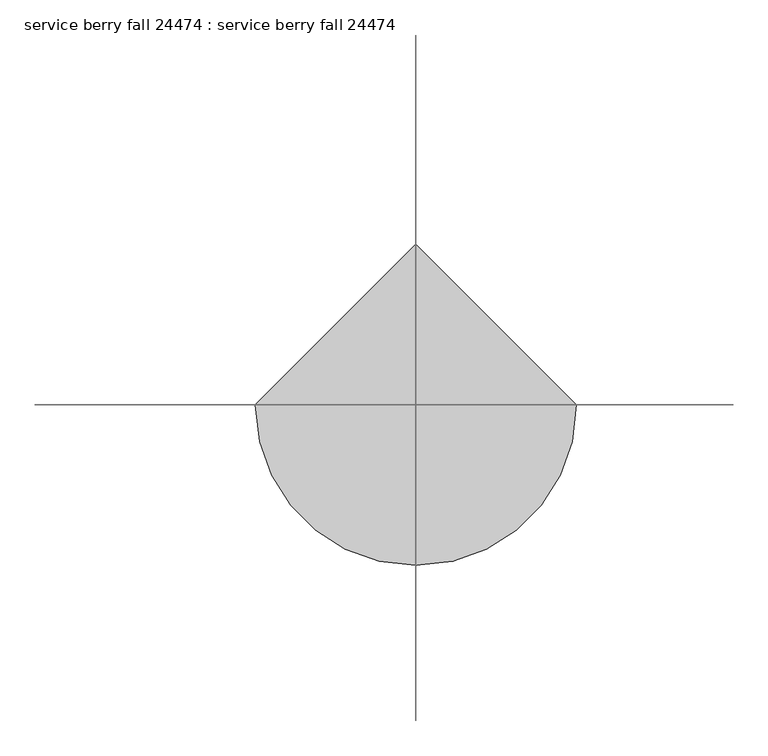
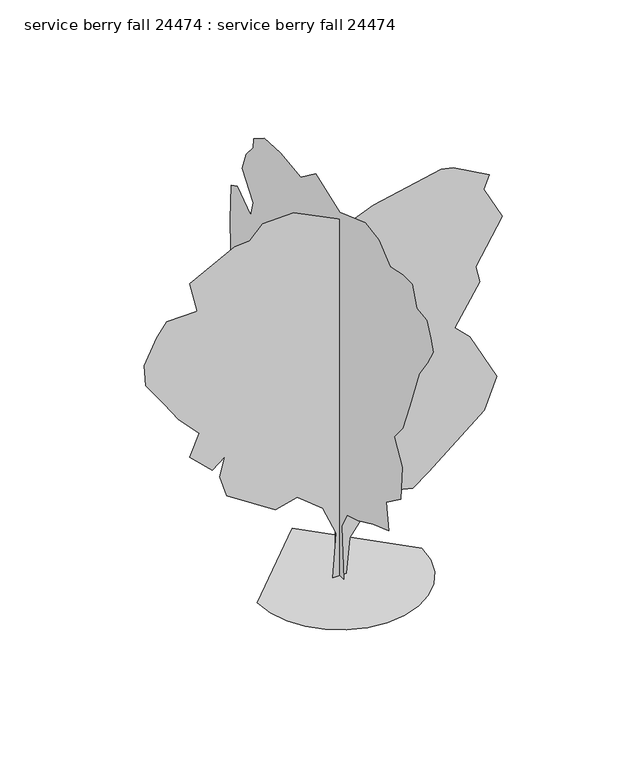
"""IFC4 building model written with IfcOpenShell, lengths in millimetres: proxy geometry, service berry fall 24474 : service berry fall 24474."""

from ifc_helpers import new_model, si_unit, origin, place, context, project, spatial, triangles, source, transform, mapped, element, save


def service_berry_fall_24474_service_berry_fall_24474_c2e3b044(model_context):
    return source(origin(), model_context, "Body", "Tessellation", [
        triangles([(-1569.2053802, 0.0, 0.0921994), (-1527.7195404, -359.5569775, 0.0921994), (-1409.5715195, -689.7541191, 0.0921994), (-1224.2203331, -981.1298658, 0.0921994), (-981.1298658, -1224.2203331, 0.0921994), (-689.7541191, -1409.5715195, 0.0921994), (-359.5569775, -1527.7195404, 0.0921994), (6.86e-05, -1569.2053802, 0.0921994), (359.5569775, -1527.7195404, 0.0921994), (689.7541191, -1409.5715195, 0.0921994), (981.1298658, -1224.2203331, 0.0921994), (1224.2229492, -981.1298658, 0.0921994), (1409.5715195, -689.7541191, 0.0921994), (1527.7195404, -359.5569775, 0.0921994), (1569.2053802, 0.0001372, 0.0921994), (-0.0002058, 1569.2053802, 0.0921994), (-1.69e-05, -141.5174793, 0.1472589), (0.0001147, -69.7424863, 1032.2016031), (0.000133, -256.3848048, 1371.9187305), (0.0001024, -615.3550266, 1474.4812202), (7.03e-05, -1115.345874, 1705.2476578), (3.21e-05, -1615.3367214, 1884.7314697), (0.0001039, -1538.4155445, 2410.3636299), (8.87e-05, -2012.7650791, 2756.5067459), (0.0001635, -2064.0477047, 3435.9815506), (0.000217, -1897.3831684, 3718.0227654), (0.0002491, -1794.8206787, 3884.6974754), (0.0002552, -2089.6888721, 4230.8484398), (0.000298, -2307.6334179, 4807.7579933), (0.0003614, -2623.385511, 5655.5326996), (0.0003744, -2884.5480583, 6025.68685), (0.0003913, -3089.67827, 6371.8378143), (0.0004295, -2999.9401428, 6602.5964035), (0.0004784, -2871.721225, 6884.6379089), (0.0005227, -2551.224218, 6935.9202438), (0.0005869, -2397.3740158, 7320.5264191), (0.0006248, -2079.5720478, 7320.8822113), (0.0006638, -1662.9541637, 7231.2458221), (0.0007467, -1282.8054199, 7546.7643539), (0.0008078, -843.8836647, 7619.9924423), (0.0008724, -0.5889314, 7319.3073074), (0.0010019, 789.2051708, 7615.6235229), (0.0010175, 1284.1033058, 7251.4131958), (0.001108, 1961.5257648, 7333.3535431), (0.0011676, 2487.1577797, 7307.7248749), (0.0011829, 2846.1178459, 7076.9407059), (0.0011624, 2859.3260513, 6891.47005), (0.0011569, 3089.7038498, 6615.4235275), (0.0011294, 3217.9227676, 6256.4454391), (0.0010299, 2847.8197769, 5791.7784531), (0.0010042, 2946.0922668, 5477.7836655), (0.0010936, 3377.5871498, 5796.1217926), (0.0011065, 3589.7021095, 5692.3630096), (0.0010255, 3615.3560669, 4987.2339569), (0.0008843, 3582.2092529, 3836.2597343), (0.0007687, 3089.7038498, 3359.0705475), (0.0006236, 2628.1860901, 2602.6591599), (0.0005208, 2040.694915, 2327.8239006), (0.0004249, 1431.5069538, 2133.0466908), (0.0004088, 1159.6180264, 2269.3404064), (0.0003546, 948.7221056, 2025.7546932), (0.0003347, 1038.465247, 1769.3469429), (0.0003041, 974.3633457, 1577.0438553), (0.0002185, 601.9539914, 1230.895507), (0.0002096, 314.8453897, 1443.1579868), (0.0001473, 143.6297414, 1092.3639919), (1.53e-05, 128.0166319, 0.0873663), (-131.1532773, 5.7e-06, 1.11e-05), (-67.2957107, -0.0001014, 875.4050692), (-322.2342556, -0.0001611, 1469.2590099), (-813.1217342, -0.0001862, 1859.996933), (-1229.3790298, -0.000155, 1751.1580822), (-2156.2470188, -0.0001869, 2358.9337749), (-2290.3894123, -0.0002327, 2792.1938118), (-2194.7076073, -0.0002815, 3166.6148529), (-2430.1146046, -0.0002486, 2976.2674599), (-2861.3579041, -0.0002784, 3384.5466087), (-2681.1450668, -0.0003364, 3804.8398499), (-3066.4881157, -0.0003688, 4217.8689995), (-3348.5293304, -0.0004053, 4628.1294228), (-3694.6802948, -0.0004483, 5115.3011398), (-3724.9569351, -0.0004968, 5533.4604996), (-3491.4551994, -0.000565, 6019.7430267), (-3297.2469955, -0.0006032, 6269.1202469), (-2715.1302017, -0.0006298, 6278.9242996), (-2861.3579041, -0.0006956, 6884.5105911), (-2002.4019035, -0.0007866, 7333.2012268), (-1714.1578697, -0.0008013, 7350.6001648), (-1463.9504677, -0.0008423, 7602.441188), (-879.4385439, -0.0008697, 7618.3158005), (233.9073432, -0.0008534, 7073.1560532), (638.5782457, -0.0008914, 7243.4630997), (1933.428352, -0.0009801, 7512.7030609), (2164.1946442, -0.0009841, 7461.4201447), (2852.671225, -0.0009686, 7079.2521927), (2750.5632133, -0.0009338, 6825.0491043), (3100.854332, -0.0008692, 6154.4644547), (2597.0202599, -0.000747, 5314.284343), (2668.3182335, -0.0007111, 4986.9549042), (2193.0693352, -0.0006001, 4229.7307755), (2484.1352898, -0.0005783, 3940.602784), (2995.342749, -0.0004845, 2966.2343513), (2760.2152405, -0.0004028, 2366.9321239), (1689.8424934, -0.0002511, 1487.1532665), (1388.3447628, -0.0002125, 1273.8112015), (830.8839495, -0.0002044, 1410.2319443), (535.8861128, -0.0001613, 1156.8088228), (193.8940152, -9.15e-05, 696.3936121), (121.4733449, -5.3e-06, 0.0)], [[15, 16, 1], [14, 15, 1], [14, 1, 2], [13, 14, 2], [13, 2, 3], [13, 3, 4], [12, 13, 4], [11, 12, 4], [11, 4, 5], [11, 5, 6], [11, 6, 7], [11, 7, 8], [11, 8, 9], [11, 9, 10], [67, 17, 18], [66, 67, 18], [63, 64, 65], [21, 22, 23], [66, 18, 19], [65, 66, 19], [35, 36, 37], [51, 52, 53], [51, 53, 54], [62, 63, 65], [61, 62, 65], [48, 49, 50], [41, 42, 43], [33, 34, 35], [47, 48, 50], [51, 54, 55], [51, 55, 56], [45, 46, 47], [31, 32, 33], [31, 33, 35], [30, 31, 35], [35, 37, 38], [30, 35, 38], [29, 30, 38], [23, 24, 25], [23, 25, 26], [23, 26, 27], [44, 45, 47], [44, 47, 50], [43, 44, 50], [58, 59, 60], [41, 43, 50], [41, 50, 51], [41, 51, 56], [41, 56, 57], [41, 57, 58], [41, 58, 60], [40, 41, 60], [39, 40, 60], [38, 39, 60], [29, 38, 60], [28, 29, 60], [27, 28, 60], [23, 27, 60], [23, 60, 61], [21, 23, 61], [20, 21, 61], [20, 61, 65], [20, 65, 19], [109, 68, 69], [108, 109, 69], [107, 108, 69], [107, 69, 70], [94, 95, 96], [75, 76, 77], [75, 77, 78], [85, 86, 87], [106, 107, 70], [96, 97, 98], [85, 87, 88], [83, 84, 85], [101, 102, 103], [101, 103, 104], [100, 101, 104], [104, 105, 106], [100, 104, 106], [100, 106, 70], [100, 70, 71], [94, 96, 98], [93, 94, 98], [92, 93, 98], [91, 92, 98], [71, 72, 73], [100, 71, 73], [100, 73, 74], [100, 74, 75], [100, 75, 78], [99, 100, 78], [98, 99, 78], [91, 98, 78], [90, 91, 78], [89, 90, 78], [88, 89, 78], [85, 88, 78], [85, 78, 79], [85, 79, 80], [83, 85, 80], [83, 80, 81], [82, 83, 81]], closed=False),
    ])


if __name__ == "__main__":
    model = new_model("IFC4")
    model_context = context("Model", 3, world=origin())
    ifc_project = project(units=[si_unit("LENGTHUNIT", "METRE", prefix="MILLI")], contexts=[model_context])
    site = spatial("IfcSite", under=ifc_project)
    building = spatial("IfcBuilding", under=site)
    placement = place(None, origin())
    service_berry_fall_24474_service_berry_fall_24474_shape = service_berry_fall_24474_service_berry_fall_24474_c2e3b044(model_context)
    element("IfcBuildingElementProxy", 1, Name="service berry fall 24474 : service berry fall 24474", ObjectType="service berry fall 24474 : service berry fall 24474", at=placement, inside=building, context=model_context, shape_type="MappedRepresentation", body=[
        mapped(service_berry_fall_24474_service_berry_fall_24474_shape, transform((0.0, 0.0, 0.0), x_axis=(1.0, 0.0, 0.0), y_axis=(0.0, 1.0, 0.0), z_axis=(0.0, 0.0, 1.0))),
    ])
    save(model, "model.ifc")

# Revit data of these elements
# Type "service berry fall 24474 : service berry fall 24474"
#   built-in parameter 1005195 = "RPC-16-FVGU-8VG0-7PL0-4000-ST1L-LVER-AU"
#   Height = 0
